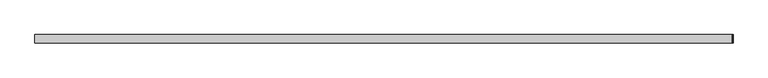
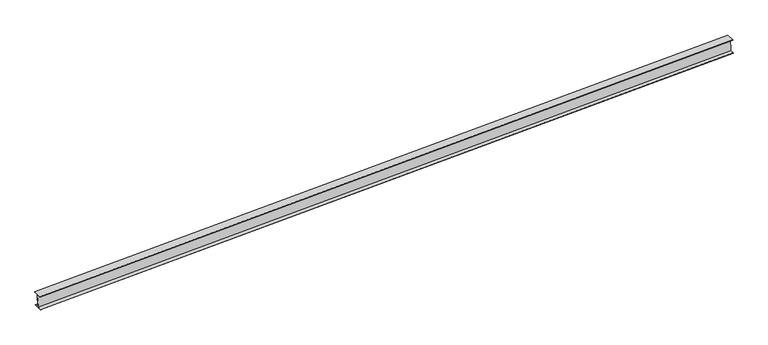
"""IFC4 building model written with IfcOpenShell, lengths in millimetres: proxy geometry, Generic Models 2:Generic Models 2:310765:Generic Models 2:310765 : Generic Models 2:Generic Models 2:310765:18 : Generic Models 2:Generic Models 2:310765:Generic Models 2:310765 : Generic Models 2:Generic Models 2:310765:300385."""

from ifc_helpers import new_model, si_unit, frame, origin, place, context, project, spatial, polyline, outline, extrude, source, transform, mapped, element, save


def generic_models_090aed6e(model_context):
    return source(origin(), model_context, "Body", "SweptSolid", [
        extrude(outline(polyline([(0.0, 0.0), (0.0, -6.858), (-152.4, -6.858), (-152.4, 0.0), (-79.121, 0.0), (-79.121, 240.2840001), (-152.4, 240.2840001), (-152.4, 247.142), (0.0, 247.142), (0.0, 240.2840001), (-73.025, 240.2840001), (-73.025, 0.0), (0.0, 0.0)])), frame((563169.680988, -578474.93331, 3820.2759387), z_axis=(0.9991330730923568, 0.0, 0.04163054471206784), x_axis=(0.0, -1.0, 0.0)), (0.0, 0.0, 1.0), 12411.242059),
    ])


if __name__ == "__main__":
    model = new_model("IFC4")
    model_context = context("Model", 3, world=origin())
    ifc_project = project(units=[si_unit("LENGTHUNIT", "METRE", prefix="MILLI")], contexts=[model_context])
    site = spatial("IfcSite", under=ifc_project)
    building = spatial("IfcBuilding", under=site)
    placement = place(None, origin())
    generic_models_shape = generic_models_090aed6e(model_context)
    element("IfcBuildingElementProxy", 1, Name="Generic Models 2:Generic Models 2:310765:Generic Models 2:310765 : Generic Models 2:Generic Models 2:310765:18 : Generic Models 2:Generic Models 2:310765:Generic Models 2:310765 : Generic Models 2:Generic Models 2:310765:300385", ObjectType="Generic Models 2:Generic Models 2:310765:Generic Models 2:310765 : Generic Models 2:Generic Models 2:310765:18 : Generic Models 2:Generic Models 2:310765:Generic Models 2:310765 : Generic Models 2:Generic Models 2:310765:300385", at=placement, inside=building, context=model_context, shape_type="MappedRepresentation", body=[
        mapped(generic_models_shape, transform((0.0, 0.0, 0.0), x_axis=(1.0, 0.0, 0.0), y_axis=(0.0, 1.0, 0.0), z_axis=(0.0, 0.0, 1.0))),
    ])
    save(model, "model.ifc")

# Revit data of these elements
# Type "Generic Models 2:Generic Models 2:310765:Generic Models 2:310765 : Generic Models 2:Generic Models 2:310765:18 : Generic Models 2:Generic Models 2:310765:Generic Models 2:310765 : Generic Models 2:Generic Models 2:310765:300385"
#   NameOverride = "Generic Models 2:Generic Models 2:310765:Generic Models 2:310765 : Generic Models 2:Generic Models 2:310765:300385"
#   ObjectTypeOverride = "Generic Models 2:310765 : Generic Models 2:Generic Models 2:310765"
#   Reference = "Generic Models 2"
#   Tag = "300385"
# Element 1 (IfcBuildingElementProxy, "Generic Models 2:Generic Models 2:310765:Generic Models 2:310765 : Generic Models 2:Generic Models 2:310765:18 : Generic Models 2:Generic Models 2:310765:Generic Models 2:310765 : Generic Models 2:Generic Models 2:310765:300385")
#   Materials on its faces: "THERMAL BROKEN ALUMINUM STOREFRONT FOR POLYCARBONATE"
# Materials
#   "THERMAL BROKEN ALUMINUM STOREFRONT FOR POLYCARBONATE": class "Unassigned", colour RGB 244 244 244, transparency 0, Keynote = "M07611300.01", Cost = 0
